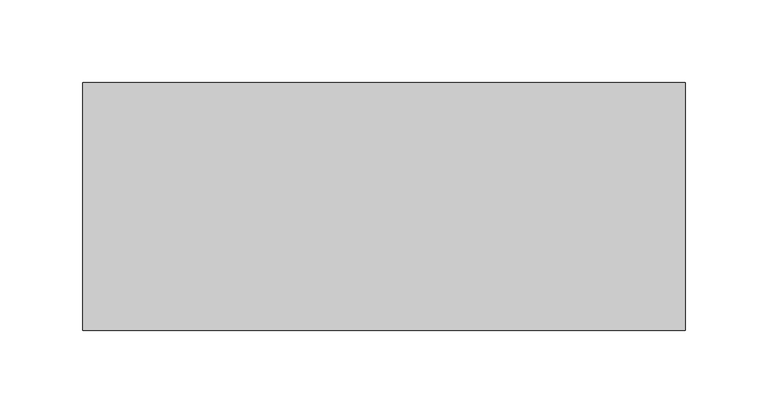
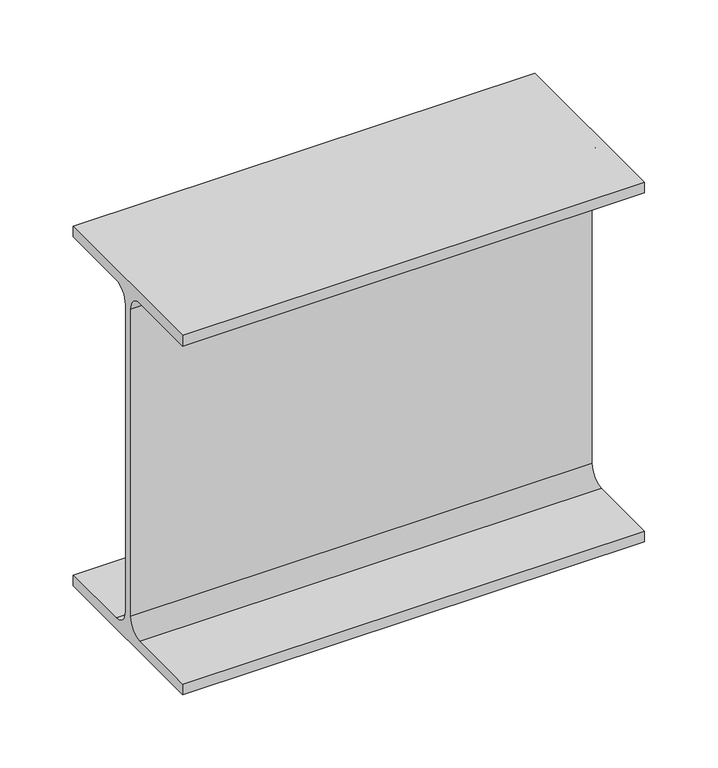
"""IFC4 building model written with IfcOpenShell, lengths in millimetres: beam geometry, 0912_Steel Framing_H-KSD3502 : H_SB_ASB_H-300x150x6.5x9."""

from ifc_helpers import new_model, si_unit, point, frame, frame_2d, origin, place, context, project, spatial, polyline, circle_curve, trimmed, segment, composite_curve, outline, extrude, source, transform, mapped, element, save


def beam_c837beb5(model_context):
    return source(origin(), model_context, "Body", "SweptSolid", [
        extrude(outline(composite_curve([segment(polyline([(75.0, -141.0), (75.0, -150.0), (-75.0, -150.0), (-75.0, -141.0), (-16.25, -141.0)]), True, "CONTINUOUS"), segment(trimmed(circle_curve(frame_2d((-16.25, -128.0)), 13.0), [point((-16.25, -141.0))], [point((-3.25, -128.0))], True, "CARTESIAN"), True, "CONTINUOUS"), segment(polyline([(-3.25, -128.0), (-3.25, 128.0)]), True, "CONTINUOUS"), segment(trimmed(circle_curve(frame_2d((-16.25, 128.0)), 13.0), [point((-3.25, 128.0))], [point((-16.25, 141.0))], True, "CARTESIAN"), True, "CONTINUOUS"), segment(polyline([(-16.25, 141.0), (-75.0, 141.0), (-75.0, 150.0), (75.0, 150.0), (75.0, 141.0), (16.25, 141.0)]), True, "CONTINUOUS"), segment(trimmed(circle_curve(frame_2d((16.25, 128.0)), 13.0), [point((16.25, 141.0))], [point((3.25, 128.0))], True, "CARTESIAN"), True, "CONTINUOUS"), segment(polyline([(3.25, 128.0), (3.25, -128.0)]), True, "CONTINUOUS"), segment(trimmed(circle_curve(frame_2d((16.25, -128.0)), 13.0), [point((3.25, -128.0))], [point((16.25, -141.0))], True, "CARTESIAN"), True, "CONTINUOUS"), segment(polyline([(16.25, -141.0), (75.0, -141.0)]), True, "CONTINUOUS")], self_intersect=False)), frame((-107.3, 0.0, 0.0), z_axis=(1.0, 0.0, 0.0), x_axis=(0.0, 1.0, 0.0)), (0.0, 0.0, 1.0), 364.5999994),
    ])


if __name__ == "__main__":
    model = new_model("IFC4")
    model_context = context("Model", 3, world=origin())
    ifc_project = project(units=[si_unit("LENGTHUNIT", "METRE", prefix="MILLI")], contexts=[model_context])
    site = spatial("IfcSite", under=ifc_project)
    building = spatial("IfcBuilding", under=site)
    placement = place(None, origin())
    beam_shape = beam_c837beb5(model_context)
    element("IfcBeam", 1, ObjectType="0912_Steel Framing_H-KSD3502 : H_SB_ASB_H-300x150x6.5x9", at=placement, inside=building, context=model_context, shape_type="MappedRepresentation", body=[
        mapped(beam_shape, transform((0.0, 0.0, 0.0), x_axis=(1.0, 0.0, 0.0), y_axis=(0.0, 1.0, 0.0), z_axis=(0.0, 0.0, 1.0))),
    ])
    save(model, "model.ifc")

# Revit data of these elements
# Type "0912_Steel Framing_H-KSD3502 : H_SB_ASB_H-300x150x6.5x9"
#   H_WM Code_1 = "S01AA002-00001 | Main Steel Structure Fabrication Work | Shelter/Building | Medium Steel - Standard (90KG/M>Weight≥30KG/M) | Material: (   )"
#   H_WM Code_2 = "S03AA028-00001 | Main Steel Structure Erection Work | Shelter/Building | Medium Steel (90KG/M>Weight≥30KG/M) | Material: (   )"
#   H_WM Code_3 = "S01AA010-00001 | Main Steel Structure Fabrication Work | Shelter/Building | Steel Painting/Coating | for Non-Fireproofed Steel Surface, Surface Preparation, Primer, Second & Final Coat | Material: (   )"
#   H_Q'ty Cal Type Tag = "SB-Q2"
#   Width = 15.0 cm
#   Web Thickness = 0.65 cm
#   Web Fillet = 1.3 cm
#   Warping Constant = 107000.0 cm⁶
#   W = 0
#   Torsional Moment of Inertia = 9.9539 cm⁴
#   Section Area = 46.78 cm²
#   Plastic Modulus weak axis = 105.0 cm³
#   Plastic Modulus strong axis = 542.0 cm³
#   Perimeter = 1.17 m²/m
#   Nominal Weight = 36.70 kgf/m
#   Moment of Inertia weak axis = 508.00 cm⁴
#   Moment of Inertia strong axis = 7210.00 cm⁴
#   Height = 30.0 cm
#   Flange Thickness = 0.9 cm
#   Elastic Modulus weak axis = 67.7 cm³
#   Elastic Modulus strong axis = 481.0 cm³
#   Centroid Vertical = 15.0 cm
#   Centroid Horizontal = 7.5 cm
#   Ix = 72100000
#   Length [instance default] = 1.5240 m
#   Zx = 542000
#   b = 0.1500 m
#   h = 0.3000 m
#   r = 0.0130 m
#   s = 0.0065 m
#   t = 0.0090 m
#   A = 0.004678 m²
#   Structural Material [instance default] = Steel, 45-345
#   Assembly Code = ""
# Element 1 (IfcBeam, "0912_Steel Framing_H-KSD3502 : H_SB_ASB_H-300x150x6.5x9")
#   Structural Material = none
# Materials
#   "Steel, 45-345": class "Metal", colour RGB 189 187 185, transparency 0, Description = "Steel 345 MPa", Cost = 0
